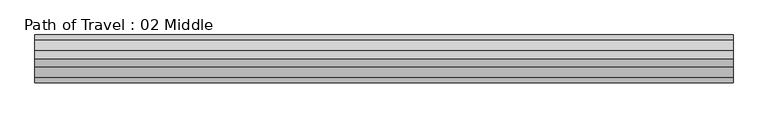
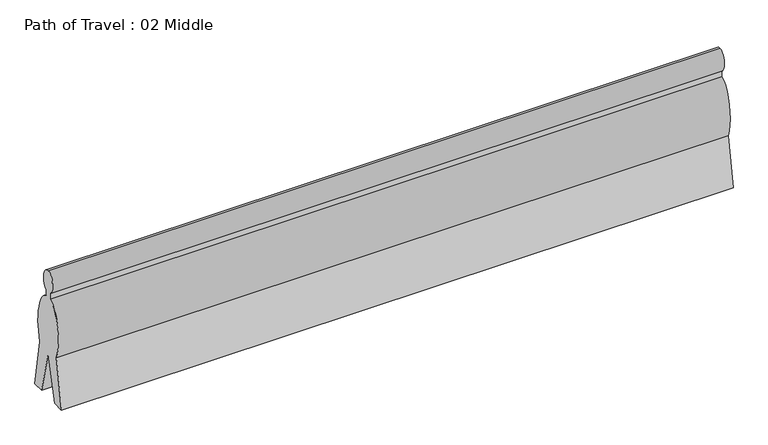
"""IFC4 building model written with IfcOpenShell, lengths in millimetres: proxy geometry, Path of Travel : 02 Middle."""

import ifcopenshell
import ifcopenshell.guid

model = None  # the IFC model being written
_history = None  # IfcOwnerHistory: only IFC2X3 demands one
_inside = {}  # id of a spatial element -> (the spatial element, [elements in it])
_under = {}  # id of a project, library or spatial element -> (it, [spatial elements below it])
_declared = {}  # id of a project -> (the project, [libraries it declares])
_typed = {}  # id of a type object -> (the type object, [elements of that type])
_made_of = {}  # id of a material, layer set ... -> (it, [elements and type objects made of it])


def new_model(schema):
    """Start an empty IFC model of exactly this schema.

    Asked for "IFC4X3", IfcOpenShell would pick the latest addendum, in which some entities
    have other attributes; the version numbers below select the first issue.
    IFC2X3 requires an IfcOwnerHistory on every rooted entity: one is made here for all.
    """
    global model, _history
    if schema == "IFC4X3":
        model = ifcopenshell.file(schema_version=(4, 3, 0, 0))
    else:
        model = ifcopenshell.file(schema=schema)
    _inside.clear()
    _under.clear()
    _declared.clear()
    _typed.clear()
    _made_of.clear()
    _history = None
    if model.schema == "IFC2X3":
        org = make("IfcOrganization", Name="unknown")
        user = make(
            "IfcPersonAndOrganization",
            ThePerson=make("IfcPerson", FamilyName="unknown"),
            TheOrganization=org,
        )
        app = make(
            "IfcApplication",
            ApplicationDeveloper=org,
            Version="unknown",
            ApplicationFullName="unknown",
            ApplicationIdentifier="unknown",
        )
        _history = make(
            "IfcOwnerHistory",
            OwningUser=user,
            OwningApplication=app,
            ChangeAction="ADDED",
            CreationDate=0,
        )
    return model


def make(cls, **values):
    """One entity of the class cls with the attributes given. An attribute that is None is left unset."""
    return model.create_entity(
        cls, **{name: value for name, value in values.items() if value is not None}
    )


def rooted(cls, **values):
    """An entity with a GlobalId (a new one), such as an element, a storey or a relation."""
    return make(cls, GlobalId=ifcopenshell.guid.new(), OwnerHistory=_history, **values)


def si_unit(unit_type, name, prefix=None):
    """IfcSIUnit, for example si_unit("LENGTHUNIT", "METRE", prefix="MILLI")."""
    return make("IfcSIUnit", UnitType=unit_type, Prefix=prefix, Name=name)


def assignment(units):
    """IfcUnitAssignment: the units of a project."""
    return None if units is None else make("IfcUnitAssignment", Units=units)


def point(xyz):
    """IfcCartesianPoint."""
    return None if xyz is None else make("IfcCartesianPoint", Coordinates=xyz)


def direction(xyz):
    """IfcDirection."""
    return None if xyz is None else make("IfcDirection", DirectionRatios=xyz)


def frame(location, z_axis=None, x_axis=None):
    """IfcAxis2Placement3D, a coordinate frame: its origin and axes. An axis left out is left unset."""
    return make(
        "IfcAxis2Placement3D",
        Location=point(location),
        Axis=direction(z_axis),
        RefDirection=direction(x_axis),
    )


def origin():
    """The frame at (0, 0, 0) with its axes left unset."""
    return frame((0.0, 0.0, 0.0))


def place(relative_to, where):
    """IfcLocalPlacement: puts the frame where relative to a parent placement (None: the world)."""
    return make(
        "IfcLocalPlacement", PlacementRelTo=relative_to, RelativePlacement=where
    )


def context(
    kind, dimensions, precision=None, world=None, true_north=None, identifier=None
):
    """IfcGeometricRepresentationContext, for example the 3D "Model" context."""
    return make(
        "IfcGeometricRepresentationContext",
        ContextIdentifier=identifier,
        ContextType=kind,
        CoordinateSpaceDimension=dimensions,
        Precision=precision,
        WorldCoordinateSystem=world,
        TrueNorth=true_north,
    )


def project(units=None, contexts=None):
    """IfcProject with its units and contexts."""
    return rooted(
        "IfcProject",
        Name="project",
        RepresentationContexts=contexts,
        UnitsInContext=assignment(units),
    )


def spatial(cls, under=None, at=None, **own):
    """A site, building, storey or space (cls), placed at a placement, below another one or the project."""
    s = rooted(cls, ObjectPlacement=at, **own)
    if under is not None:
        _under.setdefault(under.id(), (under, []))[1].append(s)
    return s


def ellipse_curve(where, semi_axis1, semi_axis2):
    """IfcEllipse in the frame where."""
    return make(
        "IfcEllipse", Position=where, SemiAxis1=semi_axis1, SemiAxis2=semi_axis2
    )


def trimmed(basis, trim1, trim2, sense, master):
    """IfcTrimmedCurve: the piece of a basis curve between two trims."""
    return make(
        "IfcTrimmedCurve",
        BasisCurve=basis,
        Trim1=trim1,
        Trim2=trim2,
        SenseAgreement=sense,
        MasterRepresentation=master,
    )


def shape(context_of_items, identifier, shape_type, items):
    """IfcShapeRepresentation: the items that make up one representation, for example the "Body"."""
    return make(
        "IfcShapeRepresentation",
        ContextOfItems=context_of_items,
        RepresentationIdentifier=identifier,
        RepresentationType=shape_type,
        Items=items,
    )


def source(mapping_origin, context_of_items, identifier, shape_type, items):
    """IfcRepresentationMap: a shape defined once, which mapped items show again and again."""
    return make(
        "IfcRepresentationMap",
        MappingOrigin=mapping_origin,
        MappedRepresentation=shape(context_of_items, identifier, shape_type, items),
    )


def transform(
    local_origin,
    x_axis=None,
    y_axis=None,
    z_axis=None,
    scale=None,
    scale2=None,
    scale3=None,
    uniform=True,
):
    """IfcCartesianTransformationOperator3D, or its non-uniform kind. x_axis, y_axis, z_axis: its Axis1, 2, 3."""
    if uniform:
        return make(
            "IfcCartesianTransformationOperator3D",
            Axis1=direction(x_axis),
            Axis2=direction(y_axis),
            LocalOrigin=point(local_origin),
            Scale=scale,
            Axis3=direction(z_axis),
        )
    return make(
        "IfcCartesianTransformationOperator3DnonUniform",
        Axis1=direction(x_axis),
        Axis2=direction(y_axis),
        LocalOrigin=point(local_origin),
        Scale=scale,
        Axis3=direction(z_axis),
        Scale2=scale2,
        Scale3=scale3,
    )


def mapped(mapping_source, mapping_target):
    """IfcMappedItem: shows the shape of a source again, moved by a transform."""
    return make(
        "IfcMappedItem", MappingSource=mapping_source, MappingTarget=mapping_target
    )


def made_of(thing, what):
    """Note that an element or type object is made of a material, layer set ...; save() writes the relation."""
    if what is not None:
        _made_of.setdefault(what.id(), (what, []))[1].append(thing)
    return thing


def element(
    cls,
    number,
    at=None,
    inside=None,
    cuts=None,
    type_object=None,
    material=None,
    context=None,
    identifier="Body",
    shape_type=None,
    held_by="IfcProductDefinitionShape",
    body=None,
    shapes=None,
    **own,
):
    """One element of the class cls, such as IfcWall. Its Tag is "e" and its number.

    at: its placement. inside: the storey or other place that contains it. cuts: it is an
    opening in that element (IfcRelVoidsElement). A single representation is given by context,
    identifier, shape_type and body (its items); several are given by shapes. held_by: the class
    of the entity that holds the representations. save() writes the other relations.
    """
    e = rooted(cls, Tag="e%d" % number, ObjectPlacement=at, **own)
    if body is not None:
        shapes = [shape(context, identifier, shape_type, body)]
    if shapes is not None:
        e.Representation = make(held_by, Representations=shapes)
    if inside is not None:
        _inside.setdefault(inside.id(), (inside, []))[1].append(e)
    if cuts is not None:
        rooted(
            "IfcRelVoidsElement", RelatingBuildingElement=cuts, RelatedOpeningElement=e
        )
    if type_object is not None:
        _typed.setdefault(type_object.id(), (type_object, []))[1].append(e)
    return made_of(e, material)


def aggregate(whole, parts):
    """IfcRelAggregates: a whole, such as a stair, and the parts it consists of."""
    return rooted("IfcRelAggregates", RelatingObject=whole, RelatedObjects=parts)


def save(model, path):
    """Write the relations noted so far, then the file.

    IfcRelAggregates (storeys below a building ...), IfcRelContainedInSpatialStructure (elements
    in a storey), IfcRelDefinesByType, IfcRelAssociatesMaterial and IfcRelDeclares: one each for
    every whole, place, type object, material and project.
    """
    for whole, parts in _under.values():
        aggregate(whole, parts)
    for where, things in _inside.values():
        rooted(
            "IfcRelContainedInSpatialStructure",
            RelatedElements=things,
            RelatingStructure=where,
        )
    for kind, things in _typed.values():
        rooted("IfcRelDefinesByType", RelatedObjects=things, RelatingType=kind)
    for what, things in _made_of.values():
        rooted("IfcRelAssociatesMaterial", RelatedObjects=things, RelatingMaterial=what)
    for by, libraries in _declared.values():
        rooted("IfcRelDeclares", RelatingContext=by, RelatedDefinitions=libraries)
    model.write(path)


def plane_surface(at):
    """IfcPlane: the flat surface through the origin of the frame at, square to its z axis."""
    return make("IfcPlane", Position=at)


def extruded_surface(curve, direction_of_extrusion, depth):
    """IfcSurfaceOfLinearExtrusion: the curve pushed along a direction by depth."""
    return make(
        "IfcSurfaceOfLinearExtrusion",
        SweptCurve=make("IfcArbitraryOpenProfileDef", ProfileType="CURVE", Curve=curve),
        ExtrudedDirection=direction(direction_of_extrusion),
        Depth=depth,
    )


def advanced_brep(points, edges, surfaces, faces):
    """IfcAdvancedBrep: a solid bounded by faces that lie on surfaces and meet in shared edges.

    An edge is (start, end): straight between two places in points (the first is 0);
    or (start, end, curve); or (start, end, curve, False) where it runs against its curve.
    A face is (place in surfaces, loops), or (place, loops, False) where it looks against
    its surface's normal. A loop lists edges by number (the first is 1), with a minus sign
    where the edge is run from its end to its start. The first loop is the outer one.
    """
    corners = [point(p) for p in points]
    vertices = [make("IfcVertexPoint", VertexGeometry=c) for c in corners]
    made = []
    for start, end, *more in edges:
        made.append(
            make(
                "IfcEdgeCurve",
                EdgeStart=vertices[start],
                EdgeEnd=vertices[end],
                EdgeGeometry=more[0] if more else make("IfcPolyline", Points=[corners[start], corners[end]]),
                SameSense=more[1] if len(more) > 1 else True,
            )
        )
    hull = []
    for where, loops, *sense in faces:
        bounds = []
        for j, loop in enumerate(loops):
            ring = [make("IfcOrientedEdge", EdgeElement=made[abs(k) - 1], Orientation=k > 0) for k in loop]
            bounds.append(
                make(
                    "IfcFaceOuterBound" if j == 0 else "IfcFaceBound",
                    Bound=make("IfcEdgeLoop", EdgeList=ring),
                    Orientation=True,
                )
            )
        hull.append(make("IfcAdvancedFace", Bounds=bounds, FaceSurface=surfaces[where], SameSense=sense[0] if sense else True))
    return make("IfcAdvancedBrep", Outer=make("IfcClosedShell", CfsFaces=hull))


def path_of_travel_02_middle_3b68c140(model_context):
    return source(origin(), model_context, "Body", "AdvancedBrep", [
        advanced_brep(
        [(227.5554837, 0.0, 1727.2), (227.5554837, 42.9018657, 1436.6534209), (227.5554837, 42.9018657, 1363.4763406), (227.5554837, 184.1186263, 643.4144547), (227.5554837, 297.5699544, 0.0), (227.5554837, 145.6574193, 0.0), (227.5554837, 0.0, 584.2), (227.5554837, -145.6574193, 0.0), (227.5554837, -297.5699544, 0.0), (227.5554837, -184.1186263, 643.4144547), (227.5554837, -42.9018657, 1363.4763406), (227.5554837, -42.9018657, 1436.6534209), (8914.3554837, 0.0, 1727.2), (8914.3554837, -42.9018657, 1436.6534209), (8914.3554837, -42.9018657, 1363.4763406), (8914.3554837, -184.1186263, 643.4144547), (8914.3554837, -297.5699544, 0.0), (8914.3554837, -145.6574193, 0.0), (8914.3554837, 0.0, 584.2), (8914.3554837, 145.6574193, 0.0), (8914.3554837, 297.5699544, 0.0), (8914.3554837, 184.1186263, 643.4144547), (8914.3554837, 42.9018657, 1363.4763406), (8914.3554837, 42.9018657, 1436.6534209)],
        [
            (0, 1, ellipse_curve(frame((227.5554837, 0.0, 1574.8), z_axis=(-1.0, 0.0, 0.0), x_axis=(0.0, 0.0, 1.0)), 152.4, 101.6)),
            (1, 2),
            (2, 3, ellipse_curve(frame((227.5554837, 0.0, 914.4), z_axis=(-1.0, 0.0, 0.0), x_axis=(0.0, 0.0, -1.0)), 457.2, 228.6)),
            (3, 4),
            (4, 5),
            (5, 6),
            (6, 7),
            (7, 8),
            (8, 9),
            (9, 10, ellipse_curve(frame((227.5554837, 0.0, 914.4), z_axis=(-1.0, 0.0, 0.0), x_axis=(0.0, 0.0, -1.0)), 457.2, 228.6)),
            (10, 11),
            (11, 0, ellipse_curve(frame((227.5554837, 0.0, 1574.8), z_axis=(-1.0, 0.0, 0.0), x_axis=(0.0, 0.0, 1.0)), 152.4, 101.6)),
            (12, 13, ellipse_curve(frame((8914.3554837, 0.0, 1574.8), z_axis=(1.0, 0.0, 0.0), x_axis=(0.0, 0.0, 1.0)), 152.4, 101.6)),
            (13, 14),
            (14, 15, ellipse_curve(frame((8914.3554837, 0.0, 914.4), z_axis=(1.0, 0.0, 0.0), x_axis=(0.0, 0.0, -1.0)), 457.2, 228.6)),
            (15, 16),
            (16, 17),
            (17, 18),
            (18, 19),
            (19, 20),
            (20, 21),
            (21, 22, ellipse_curve(frame((8914.3554837, 0.0, 914.4), z_axis=(1.0, 0.0, 0.0), x_axis=(0.0, 0.0, -1.0)), 457.2, 228.6)),
            (22, 23),
            (23, 12, ellipse_curve(frame((8914.3554837, 0.0, 1574.8), z_axis=(1.0, 0.0, 0.0), x_axis=(0.0, 0.0, 1.0)), 152.4, 101.6)),
            (0, 12),
            (23, 1),
            (22, 2),
            (21, 3),
            (20, 4),
            (19, 5),
            (18, 6),
            (17, 7),
            (16, 8),
            (15, 9),
            (14, 10),
            (13, 11),
        ],
        [
            plane_surface(frame((227.5554837, 0.0, 0.0), z_axis=(-1.0, 0.0, 0.0), x_axis=(0.0, 0.0, 1.0))),
            plane_surface(frame((8914.3554837, 0.0, 0.0), z_axis=(1.0, 0.0, 0.0), x_axis=(0.0, 0.0, 1.0))),
            extruded_surface(trimmed(ellipse_curve(frame((8914.3554837, 0.0, 1574.8), z_axis=(-1.0, 0.0, 0.0), x_axis=(0.0, 0.0, 1.0)), 152.4, 101.6), [point((8914.3554837, 0.0, 1727.2))], [point((8914.3554837, 42.9018657, 1436.6534209))], True, "CARTESIAN"), (-8686.8, 0.0, 0.0), 8686.8),
            plane_surface(frame((227.5554837, 42.9018657, 1436.6534209), z_axis=(0.0, 1.0, 0.0), x_axis=(1.0, 0.0, 0.0))),
            extruded_surface(trimmed(ellipse_curve(frame((8914.3554837, 0.0, 914.4), z_axis=(-1.0, 0.0, 0.0), x_axis=(0.0, 0.0, -1.0)), 457.2, 228.6), [point((8914.3554837, 42.9018657, 1363.4763406))], [point((8914.3554837, 184.1186263, 643.4144547))], True, "CARTESIAN"), (-8686.8, 0.0, 0.0), 8686.8),
            plane_surface(frame((227.5554837, 184.1186263, 643.4144547), z_axis=(0.0, 0.9848077530122078, 0.17364817766693205), x_axis=(1.0, 0.0, 0.0))),
            plane_surface(frame((227.5554837, 297.5699544, 0.0), z_axis=(0.0, 0.0, -1.0), x_axis=(1.0, 0.0, 0.0))),
            plane_surface(frame((227.5554837, 145.6574193, 0.0), z_axis=(0.0, -0.9702957262760199, -0.2419218955995739), x_axis=(1.0, 0.0, 0.0))),
            plane_surface(frame((227.5554837, 0.0, 584.2), z_axis=(0.0, 0.9702957262759961, -0.24192189559966923), x_axis=(1.0, 0.0, 0.0))),
            plane_surface(frame((227.5554837, -145.6574193, 0.0), z_axis=(0.0, 0.0, -1.0), x_axis=(1.0, 0.0, 0.0))),
            plane_surface(frame((227.5554837, -297.5699544, 0.0), z_axis=(0.0, -0.984807753012208, 0.17364817766693066), x_axis=(1.0, 0.0, 0.0))),
            extruded_surface(trimmed(ellipse_curve(frame((8914.3554837, 0.0, 914.4), z_axis=(-1.0, 0.0, 0.0), x_axis=(0.0, 0.0, -1.0)), 457.2, 228.6), [point((8914.3554837, -184.1186263, 643.4144547))], [point((8914.3554837, -42.9018657, 1363.4763406))], True, "CARTESIAN"), (-8686.8, 0.0, 0.0), 8686.8),
            plane_surface(frame((227.5554837, -42.9018657, 1363.4763406), z_axis=(0.0, -1.0, 0.0), x_axis=(1.0, 0.0, 0.0))),
            extruded_surface(trimmed(ellipse_curve(frame((8914.3554837, 0.0, 1574.8), z_axis=(-1.0, 0.0, 0.0), x_axis=(0.0, 0.0, 1.0)), 152.4, 101.6), [point((8914.3554837, -42.9018657, 1436.6534209))], [point((8914.3554837, 0.0, 1727.2))], True, "CARTESIAN"), (-8686.8, 0.0, 0.0), 8686.8),
        ],
        [
            (0, [[1, 2, 3, 4, 5, 6, 7, 8, 9, 10, 11, 12]]),
            (1, [[13, 14, 15, 16, 17, 18, 19, 20, 21, 22, 23, 24]]),
            (2, [[-1, 25, -24, 26]]),
            (3, [[-2, -26, -23, 27]]),
            (4, [[-3, -27, -22, 28]]),
            (5, [[-4, -28, -21, 29]]),
            (6, [[-5, -29, -20, 30]]),
            (7, [[-6, -30, -19, 31]]),
            (8, [[-7, -31, -18, 32]]),
            (9, [[-8, -32, -17, 33]]),
            (10, [[-9, -33, -16, 34]]),
            (11, [[-10, -34, -15, 35]]),
            (12, [[-11, -35, -14, 36]]),
            (13, [[-12, -36, -13, -25]]),
        ],
    ),
    ])


if __name__ == "__main__":
    model = new_model("IFC4")
    model_context = context("Model", 3, world=origin())
    ifc_project = project(units=[si_unit("LENGTHUNIT", "METRE", prefix="MILLI")], contexts=[model_context])
    site = spatial("IfcSite", under=ifc_project)
    building = spatial("IfcBuilding", under=site)
    placement = place(None, origin())
    path_of_travel_02_middle_shape = path_of_travel_02_middle_3b68c140(model_context)
    element("IfcBuildingElementProxy", 1, Name="Path of Travel : 02 Middle", ObjectType="Path of Travel : 02 Middle", at=placement, inside=building, context=model_context, shape_type="MappedRepresentation", body=[
        mapped(path_of_travel_02_middle_shape, transform((0.0, 0.0, 0.0), x_axis=(1.0, 0.0, 0.0), y_axis=(0.0, 1.0, 0.0), z_axis=(0.0, 0.0, 1.0))),
    ])
    save(model, "model.ifc")

# Revit data of these elements
# Type "Path of Travel : 02 Middle"
#   Path of Egress [instance default] = 4' - 0"
#   built-in parameter 1001306 [instance default] = 4 (stored number, unit not read)
#   Dot at Start = no
#   Arrow in Middle = yes
#   Arrow at End = no
#   Egress Path = none
# Element 1 (IfcBuildingElementProxy, "Path of Travel : 02 Middle")
#   Path of Egress = 28' - 6"
#   built-in parameter 1001306 = 28.5 (stored number, unit not read)
#   Materials on its faces: "Egress Path Solid"
# Materials
#   "Egress Path Solid": class "Unassigned", colour RGB 255 128 64, transparency 0.75, Comments = "Rendering appearance not upgraded "
